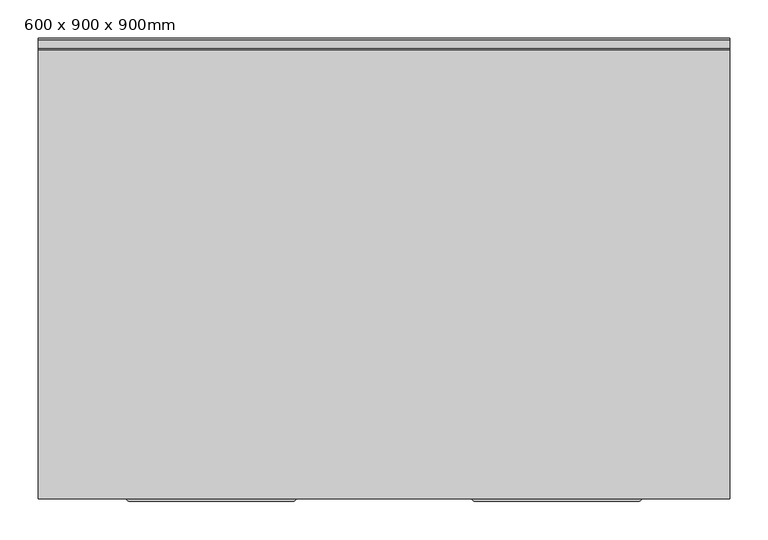
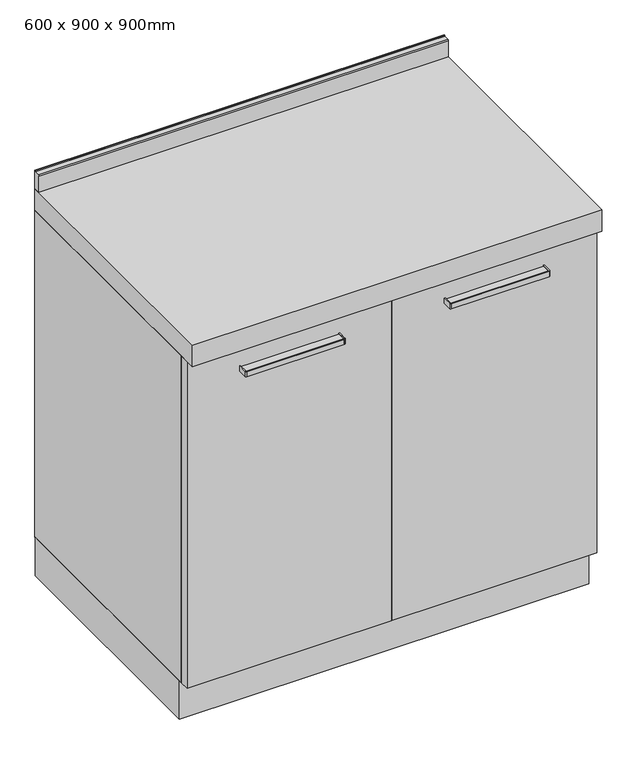
"""IFC4 building model written with IfcOpenShell, lengths in millimetres: furniture geometry, Küchenelement (1) - 2-flg : 600 x 900 x 900mm."""

from ifc_helpers import new_model, si_unit, point, frame, frame_2d, origin, origin_with_axes, place, context, project, spatial, polyline, circle_curve, trimmed, segment, composite_curve, outline, extrude, source, transform, mapped, element, save


def furniture_600_x_900_x_900mm_8fb8675d(model_context):
    return source(origin(), model_context, "Body", "SweptSolid", [
        extrude(outline(composite_curve([segment(polyline([(161.7003264, -580.0), (377.7003264, -580.0), (377.7003264, -600.5)]), True, "CONTINUOUS"), segment(trimmed(circle_curve(frame_2d((377.2003264, -600.5)), 0.5), [point((377.7003264, -600.5))], [point((377.2003264, -601.0))], False, "CARTESIAN"), True, "CONTINUOUS"), segment(polyline([(377.2003264, -601.0), (162.2003264, -601.0)]), True, "CONTINUOUS"), segment(trimmed(circle_curve(frame_2d((162.2003264, -600.5)), 0.5), [point((162.2003264, -601.0))], [point((161.7003264, -600.5))], False, "CARTESIAN"), True, "CONTINUOUS"), segment(polyline([(161.7003264, -600.5), (161.7003264, -580.0)]), True, "CONTINUOUS")], self_intersect=False)), frame((0.0, 0.0, 789.965389), z_axis=(0.0, 0.0, 1.0), x_axis=(1.0, 0.0, 0.0)), (0.0, 0.0, 1.0), 6.4890959),
        extrude(outline(composite_curve([segment(polyline([(159.7003264, -580.0), (161.7003264, -580.0), (161.7003264, -600.5)]), True, "CONTINUOUS"), segment(trimmed(circle_curve(frame_2d((162.2003264, -600.5)), 0.5), [point((161.7003264, -600.5))], [point((162.2003264, -601.0))], True, "CARTESIAN"), True, "CONTINUOUS"), segment(polyline([(162.2003264, -601.0), (377.2003264, -601.0)]), True, "CONTINUOUS"), segment(trimmed(circle_curve(frame_2d((377.2003264, -600.5)), 0.5), [point((377.2003264, -601.0))], [point((377.7003264, -600.5))], True, "CARTESIAN"), True, "CONTINUOUS"), segment(polyline([(377.7003264, -600.5), (377.7003264, -580.0), (379.7003264, -580.0), (379.7003264, -600.5)]), True, "CONTINUOUS"), segment(trimmed(circle_curve(frame_2d((377.2003264, -600.5)), 2.5), [point((379.7003264, -600.5))], [point((377.2003264, -603.0))], False, "CARTESIAN"), True, "CONTINUOUS"), segment(polyline([(377.2003264, -603.0), (162.2003264, -603.0)]), True, "CONTINUOUS"), segment(trimmed(circle_curve(frame_2d((162.2003264, -600.5)), 2.5), [point((162.2003264, -603.0))], [point((159.7003264, -600.5))], False, "CARTESIAN"), True, "CONTINUOUS"), segment(polyline([(159.7003264, -600.5), (159.7003264, -580.0)]), True, "CONTINUOUS")], self_intersect=False)), frame((0.0, 0.0, 787.2), z_axis=(0.0, 0.0, 1.0), x_axis=(1.0, 0.0, 0.0)), (0.0, 0.0, 1.0), 12.0),
        extrude(outline(composite_curve([segment(polyline([(-288.2996736, -580.0), (-72.2996736, -580.0), (-72.2996736, -600.5)]), True, "CONTINUOUS"), segment(trimmed(circle_curve(frame_2d((-72.7996736, -600.5)), 0.5), [point((-72.2996736, -600.5))], [point((-72.7996736, -601.0))], False, "CARTESIAN"), True, "CONTINUOUS"), segment(polyline([(-72.7996736, -601.0), (-287.7996736, -601.0)]), True, "CONTINUOUS"), segment(trimmed(circle_curve(frame_2d((-287.7996736, -600.5)), 0.5), [point((-287.7996736, -601.0))], [point((-288.2996736, -600.5))], False, "CARTESIAN"), True, "CONTINUOUS"), segment(polyline([(-288.2996736, -600.5), (-288.2996736, -580.0)]), True, "CONTINUOUS")], self_intersect=False)), frame((0.0, 0.0, 789.965389), z_axis=(0.0, 0.0, 1.0), x_axis=(1.0, 0.0, 0.0)), (0.0, 0.0, 1.0), 6.4890959),
        extrude(outline(composite_curve([segment(polyline([(-290.2996736, -580.0), (-288.2996736, -580.0), (-288.2996736, -600.5)]), True, "CONTINUOUS"), segment(trimmed(circle_curve(frame_2d((-287.7996736, -600.5)), 0.5), [point((-288.2996736, -600.5))], [point((-287.7996736, -601.0))], True, "CARTESIAN"), True, "CONTINUOUS"), segment(polyline([(-287.7996736, -601.0), (-72.7996736, -601.0)]), True, "CONTINUOUS"), segment(trimmed(circle_curve(frame_2d((-72.7996736, -600.5)), 0.5), [point((-72.7996736, -601.0))], [point((-72.2996736, -600.5))], True, "CARTESIAN"), True, "CONTINUOUS"), segment(polyline([(-72.2996736, -600.5), (-72.2996736, -580.0), (-70.2996736, -580.0), (-70.2996736, -600.5)]), True, "CONTINUOUS"), segment(trimmed(circle_curve(frame_2d((-72.7996736, -600.5)), 2.5), [point((-70.2996736, -600.5))], [point((-72.7996736, -603.0))], False, "CARTESIAN"), True, "CONTINUOUS"), segment(polyline([(-72.7996736, -603.0), (-287.7996736, -603.0)]), True, "CONTINUOUS"), segment(trimmed(circle_curve(frame_2d((-287.7996736, -600.5)), 2.5), [point((-287.7996736, -603.0))], [point((-290.2996736, -600.5))], False, "CARTESIAN"), True, "CONTINUOUS"), segment(polyline([(-290.2996736, -600.5), (-290.2996736, -580.0)]), True, "CONTINUOUS")], self_intersect=False)), frame((0.0, 0.0, 787.2), z_axis=(0.0, 0.0, 1.0), x_axis=(1.0, 0.0, 0.0)), (0.0, 0.0, 1.0), 12.0),
        extrude(outline(composite_curve([segment(polyline([(0.0, 942.0034681), (0.0, 900.0), (-15.0, 900.0), (-15.0, 938.0)]), True, "CONTINUOUS"), segment(trimmed(circle_curve(frame_2d((-13.0, 938.0)), 2.0), [point((-15.0, 938.0))], [point((-13.0, 940.0))], False, "CARTESIAN"), True, "CONTINUOUS"), segment(polyline([(-13.0, 940.0), (-1.50449, 940.0), (-1.50449, 942.0034681), (0.0, 942.0034681)]), True, "CONTINUOUS")], self_intersect=False)), frame((-405.2996736, 0.0, 0.0), z_axis=(1.0, 0.0, 0.0), x_axis=(0.0, 1.0, 0.0)), (0.0, 0.0, 1.0), 900.0),
        extrude(outline(polyline([(494.7003264, -0.533703), (494.7003264, -550.533703), (-405.2996736, -550.533703), (-405.2996736, -0.533703), (494.7003264, -0.533703)])), origin_with_axes(), (0.0, 0.0, 1.0), 90.0),
        extrude(outline(polyline([(494.7003264, 0.0), (494.7003264, -600.0), (-405.2996736, -600.0), (-405.2996736, 0.0), (494.7003264, 0.0)])), frame((0.0, 0.0, 850.0), z_axis=(0.0, 0.0, 1.0), x_axis=(1.0, 0.0, 0.0)), (0.0, 0.0, 1.0), 50.0),
        extrude(outline(polyline([(43.7003264, -580.0), (-405.2996736, -580.0), (-405.2996736, -558.0), (43.7003264, -558.0), (43.7003264, -580.0)])), frame((0.0, 0.0, 90.0), z_axis=(0.0, 0.0, 1.0), x_axis=(1.0, 0.0, 0.0)), (0.0, 0.0, 1.0), 760.0),
        extrude(outline(polyline([(45.7003264, -580.0), (45.7003264, -558.0), (494.7003264, -558.0), (494.7003264, -580.0), (45.7003264, -580.0)])), frame((0.0, 0.0, 90.0), z_axis=(0.0, 0.0, 1.0), x_axis=(1.0, 0.0, 0.0)), (0.0, 0.0, 1.0), 760.0),
        extrude(outline(polyline([(494.7003264, 0.0), (494.7003264, -558.0), (472.7003264, -558.0), (472.7003264, -22.0), (-383.2996736, -22.0), (-383.2996736, -558.0), (-405.2996736, -558.0), (-405.2996736, 0.0), (494.7003264, 0.0)])), frame((0.0, 0.0, 90.0), z_axis=(0.0, 0.0, 1.0), x_axis=(1.0, 0.0, 0.0)), (0.0, 0.0, 1.0), 760.0),
    ])


if __name__ == "__main__":
    model = new_model("IFC4")
    model_context = context("Model", 3, world=origin())
    ifc_project = project(units=[si_unit("LENGTHUNIT", "METRE", prefix="MILLI")], contexts=[model_context])
    site = spatial("IfcSite", under=ifc_project)
    building = spatial("IfcBuilding", under=site)
    placement = place(None, origin())
    furniture_600_x_900_x_900mm_shape = furniture_600_x_900_x_900mm_8fb8675d(model_context)
    element("IfcFurniture", 1, ObjectType="Küchenelement (1) - 2-flg : 600 x 900 x 900mm", at=placement, inside=building, context=model_context, shape_type="MappedRepresentation", body=[
        mapped(furniture_600_x_900_x_900mm_shape, transform((0.0, 0.0, 0.0), x_axis=(1.0, 0.0, 0.0), y_axis=(0.0, 1.0, 0.0), z_axis=(0.0, 0.0, 1.0))),
    ])
    save(model, "model.ifc")

# Revit data of these elements
# Type "Küchenelement (1) - 2-flg : 600 x 900 x 900mm"
#   Länge 1 = 0.1008 m
#   Depth = 0.600 m
#   Height = 0.900 m
#   Width = 0.900 m
#   Obermaterial = none
#   Material = none
#   Griffmaterial = none
#   Assembly Code = ""
# Element 1 (IfcFurniture, "Küchenelement (1) - 2-flg : 600 x 900 x 900mm")
#   Materials on its faces: "Holz - Birke"
# Materials
#   "Holz - Birke": class "Holz", colour RGB 213 164 103, transparency 0, Cost = 0
